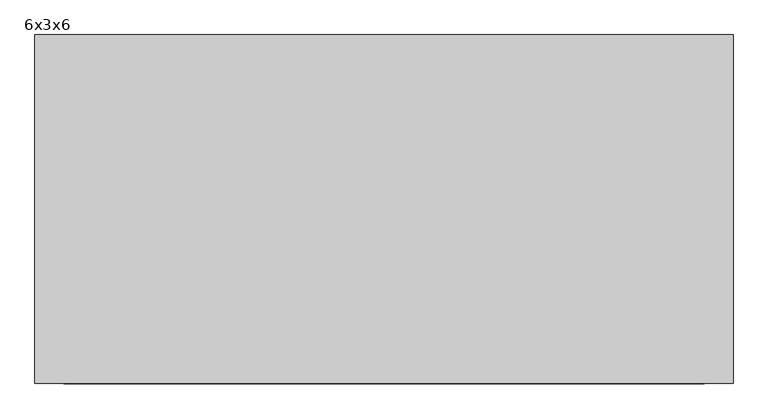
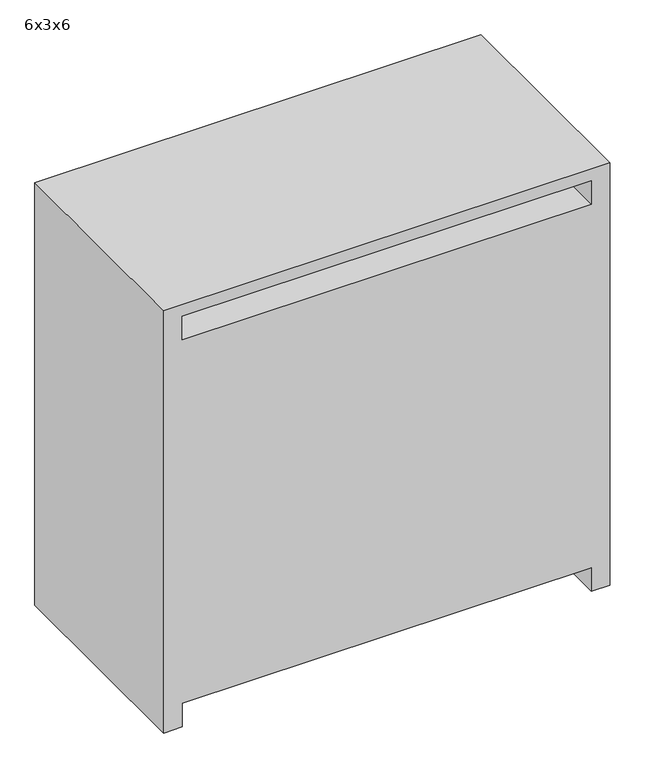
"""IFC4 building model written with IfcOpenShell, lengths in millimetres: proxy geometry, Transformer-Dry-Type-Siemens : 6x3x6."""

from ifc_helpers import new_model, si_unit, frame, origin, place, context, project, spatial, polyline, outline, extrude, source, transform, mapped, element, save


def proxy_6x3x6_82179be8(model_context):
    return source(origin(), model_context, "Body", "SweptSolid", [
        extrude(outline(polyline([(1828.8, 914.4), (1828.8, -914.4), (0.0, -914.4), (0.0, -838.2), (101.6, -838.2), (101.6, 838.2), (0.0, 838.2), (0.0, 914.4), (1828.8, 914.4)]), holes=[polyline([(1778.0, 838.2), (1676.4, 838.2), (1676.4, -838.2), (1778.0, -838.2), (1778.0, 838.2)])]), frame((0.0, -457.2, 0.0), z_axis=(0.0, 1.0, 0.0), x_axis=(0.0, 0.0, 1.0)), (0.0, 0.0, 1.0), 914.4),
    ])


if __name__ == "__main__":
    model = new_model("IFC4")
    model_context = context("Model", 3, world=origin())
    ifc_project = project(units=[si_unit("LENGTHUNIT", "METRE", prefix="MILLI")], contexts=[model_context])
    site = spatial("IfcSite", under=ifc_project)
    building = spatial("IfcBuilding", under=site)
    placement = place(None, origin())
    proxy_6x3x6_shape = proxy_6x3x6_82179be8(model_context)
    element("IfcBuildingElementProxy", 1, Name="Transformer-Dry-Type-Siemens : 6x3x6", ObjectType="Transformer-Dry-Type-Siemens : 6x3x6", at=placement, inside=building, context=model_context, shape_type="MappedRepresentation", body=[
        mapped(proxy_6x3x6_shape, transform((0.0, 0.0, 0.0), x_axis=(1.0, 0.0, 0.0), y_axis=(0.0, 1.0, 0.0), z_axis=(0.0, 0.0, 1.0))),
    ])
    save(model, "model.ifc")

# Revit data of these elements
# Type "Transformer-Dry-Type-Siemens : 6x3x6"
#   Weight = "5500"
#   Wattage = "DO NOT USE"
#   Voltage = "DO NOT USE"
#   URL = "http://www.usa.siemens.com/ce"
#   Transformer Material = "Aluminum"
#   Product Page URL = "http://www.sea.siemens.com/us/Products/PowerDistribution/Product/Transformers/Pages/Transformers.aspx"
#   Product Documentation Link = "http://www.sea.siemens.com/us/internet-dms/Internet/ConsultingEngineersComm/General/Docs/drytrans.pdf"
#   Model = "3F3Y015K13TP1"
#   Manufacturer = "Siemens Industry"
#   KVA = "750"
#   K Factor = "13"
#   Description = "Transformer"
#   Deg Rise = "150"
#   Copyright © = "© Siemens Industry, Inc. 2011"
#   CTRL Connector Description = "Equipment Power"
#   BOM URL [instance default] = ""
#   Assembly Code = "D5090900"
#   clearance = 3' - 0"
#   Width = 6' - 0"
#   Primary Voltage = 480 V
#   Power Factor = 1
#   Height = 6' - 0"
#   Depth = 3' - 0"
#   Apparent Load [instance default] = 0 VA
#   Has Not Contacted Siemens For Configuration [instance default] = no
#   Contacted Siemens For Configuration [instance default] = yes
#   Text Material = Paint- Siemens - Dark
#   Frame Material = Metal - Siemens - Steel
# Element 1 (IfcBuildingElementProxy, "Transformer-Dry-Type-Siemens : 6x3x6")
#   Materials on its faces: "Metal - Siemens - Steel"
# Materials
#   "Paint- Siemens - Dark": class "Metal", colour RGB 175 38 68, transparency 0
#   "Metal - Siemens - Steel": class "Metal", colour RGB 63 114 97, transparency 0, Cost = 0
